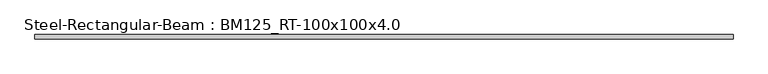
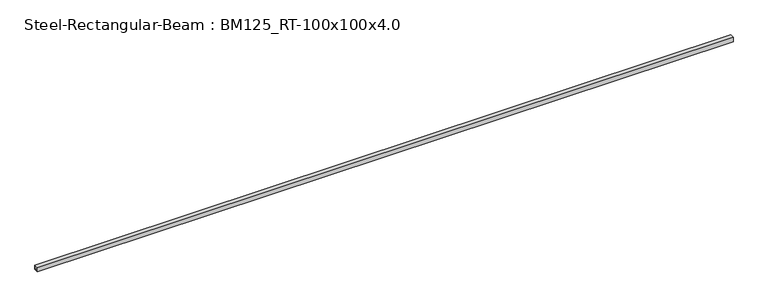
"""IFC4 building model written with IfcOpenShell, lengths in millimetres: beam geometry, Steel-Rectangular-Beam : BM125_RT-100x100x4.0."""

from ifc_helpers import new_model, si_unit, frame, origin, place, context, project, spatial, polyline, outline, extrude, source, transform, mapped, element, save


def steel_rectangular_beam_bm125_rt_100x100x4_0_fd47acba(model_context):
    return source(origin(), model_context, "Body", "SweptSolid", [
        extrude(outline(polyline([(-50.0, 50.0), (50.0, 50.0), (50.0, -50.0), (-50.0, -50.0), (-50.0, 50.0)]), holes=[polyline([(46.0, -46.0), (46.0, 46.0), (-46.0, 46.0), (-46.0, -46.0), (46.0, -46.0)])]), frame((-7887.3, 0.0, 0.0), z_axis=(1.0, 0.0, 0.0), x_axis=(0.0, 1.0, 0.0)), (0.0, 0.0, 1.0), 15774.6),
        extrude(outline(polyline([(-50.0, 50.0), (50.0, 50.0), (50.0, -50.0), (-50.0, -50.0), (-50.0, 50.0)]), holes=[polyline([(46.0, -46.0), (46.0, 46.0), (-46.0, 46.0), (-46.0, -46.0), (46.0, -46.0)])]), frame((-7887.3, 0.0, 0.0), z_axis=(1.0, 0.0, 0.0), x_axis=(0.0, 1.0, 0.0)), (0.0, 0.0, 1.0), 15774.6),
        extrude(outline(polyline([(-50.0, 50.0), (50.0, 50.0), (50.0, -50.0), (-50.0, -50.0), (-50.0, 50.0)]), holes=[polyline([(46.0, -46.0), (46.0, 46.0), (-46.0, 46.0), (-46.0, -46.0), (46.0, -46.0)])]), frame((-7887.3, 0.0, 0.0), z_axis=(1.0, 0.0, 0.0), x_axis=(0.0, 1.0, 0.0)), (0.0, 0.0, 1.0), 15774.6),
        extrude(outline(polyline([(-50.0, 50.0), (50.0, 50.0), (50.0, -50.0), (-50.0, -50.0), (-50.0, 50.0)]), holes=[polyline([(46.0, -46.0), (46.0, 46.0), (-46.0, 46.0), (-46.0, -46.0), (46.0, -46.0)])]), frame((-7887.3, 0.0, 0.0), z_axis=(1.0, 0.0, 0.0), x_axis=(0.0, 1.0, 0.0)), (0.0, 0.0, 1.0), 15774.6),
    ])


if __name__ == "__main__":
    model = new_model("IFC4")
    model_context = context("Model", 3, world=origin())
    ifc_project = project(units=[si_unit("LENGTHUNIT", "METRE", prefix="MILLI")], contexts=[model_context])
    site = spatial("IfcSite", under=ifc_project)
    building = spatial("IfcBuilding", under=site)
    placement = place(None, origin())
    steel_rectangular_beam_bm125_rt_100x100x4_0_shape = steel_rectangular_beam_bm125_rt_100x100x4_0_fd47acba(model_context)
    element("IfcBeam", 1, ObjectType="Steel-Rectangular-Beam : BM125_RT-100x100x4.0", at=placement, inside=building, context=model_context, shape_type="MappedRepresentation", body=[
        mapped(steel_rectangular_beam_bm125_rt_100x100x4_0_shape, transform((0.0, 0.0, 0.0), x_axis=(1.0, 0.0, 0.0), y_axis=(0.0, 1.0, 0.0), z_axis=(0.0, 0.0, 1.0))),
    ])
    save(model, "model.ifc")

# Revit data of these elements
# Type "Steel-Rectangular-Beam : BM125_RT-100x100x4.0"
#   t = 4 mm
#   Mass per Unit Length = 11.70 kg/m
#   Surface Area = 0.386 m²/m
#   Sectional Area = 14.95 cm²
#   Length [instance default] = 3000 mm
#   H = 100 mm
#   B = 100 mm
#   hec_material4 [instance default] = none
#   hec_material3 [instance default] = none
#   hec_material2 [instance default] = none
#   hec_material1 [instance default] = none
#   Structural Material [instance default] = none
# Element 1 (IfcBeam, "Steel-Rectangular-Beam : BM125_RT-100x100x4.0")
#   hec_material2 = S01AA010-00001_Main Steel Structure Fabrication Work_Shelter/Building_Steel Painting/Coating_for Non-Fireproofed Steel Surface, Surface Preparation, Primer, Second & Final Coat
#   hec_material1 = S03AA007-00001_Main Steel Structure Erection Work_Girth & Purlin
#   Structural Material = S01AA007-00001_Main Steel Structure Fabrication Work_Shelter/Building_Girth & Purlin
#   Materials on its faces: "S01AA010-00001_Main Steel Structure Fabrication Work_Shelter/Building_Steel Painting/Coating_for Non-Fireproofed Steel Surface, Surface Preparation, Primer, Second & Final Coat"
# Materials
#   "S01AA010-00001_Main Steel Structure Fabrication Work_Shelter/Building_Steel Painting/Coating_for Non-Fireproofed Steel Surface, Surface Preparation, Primer, Second & Final Coat": class "Metal", colour RGB 120 120 120, transparency 0, Description = "Paint finished steel", W00) Work Master Code = "S01AA010-00001", W01) Work Master_Lv1 = "Main Steel Structure Fabrication Work", W02) Work Master_Lv2 = "Shelter/Building", W03) Work Master_Spec.1 = "Steel Painting/Coating", W04) Work Master_Spec.2 = "for Non-Fireproofed Steel Surface, Surface Preparation, Primer, Second & Final Coat", Cost = 0
#   "S03AA007-00001_Main Steel Structure Erection Work_Girth & Purlin": class "Metal", colour RGB 120 120 120, transparency 0, Comments = "(30KG/M>Weight)", Description = "Structural steel 50ksi", W00) Work Master Code = "S03AA007-00001", W01) Work Master_Lv1 = "Main Steel Structure Erection Work", W02) Work Master_Lv2 = "Shelter/Building", W03) Work Master_Spec.1 = "Girth & Purlin", Cost = 0
#   "S01AA007-00001_Main Steel Structure Fabrication Work_Shelter/Building_Girth & Purlin": class "Metal", colour RGB 120 120 120, transparency 0, Comments = "(30KG/M>Weight)", Description = "Structural steel 50ksi", W00) Work Master Code = "S01AA007-00001", W01) Work Master_Lv1 = "Main Steel Structure Fabrication Work", W02) Work Master_Lv2 = "Shelter/Building", W03) Work Master_Spec.1 = "Girth & Purlin", Cost = 0
